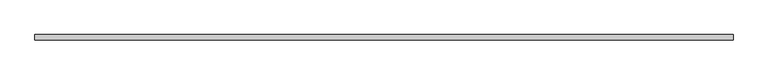
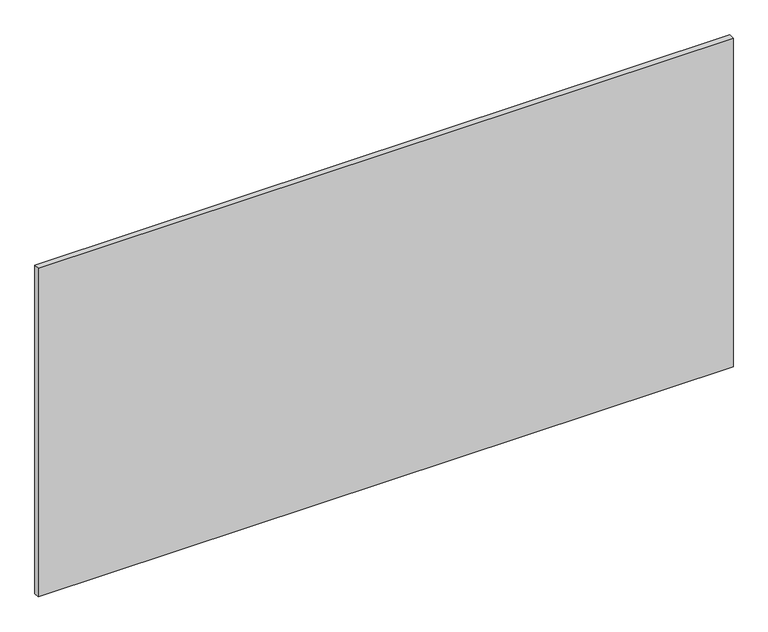
"""IFC4 building model written with IfcOpenShell, lengths in millimetres: proxy geometry, Inner panel:Inner panel:1:Inner panel:1 : Inner panel:Inner panel:300324:300043:Inner panel:1:Inner panel:1 : Inner panel:Inner panel:300324:300043 : Inner panel:Inner panel:1:Inner panel:1 : Inner panel:Inner panel:300324:300043:22 : Inner panel:Inner panel:1:Inner panel:1 : Inner panel:Inner panel:300324:300043:Inner panel:1:Inner panel:1 : Inner panel:Inner panel:300324:300043 : Inner panel:Inner panel:1:Inner panel:1 : Inner panel:Inner panel:300324:300043:300031."""

from ifc_helpers import new_model, si_unit, frame, origin, place, context, project, spatial, polyline, outline, extrude, source, transform, mapped, element, save


def generic_models_5df29abb(model_context):
    return source(origin(), model_context, "Body", "SweptSolid", [
        extrude(outline(polyline([(593738.0867239, -567913.5913841), (596176.4867239, -567913.5913841), (596176.4867239, -567932.6413841), (593738.0867239, -567932.6413841), (593738.0867239, -567913.5913841)])), frame((0.0, 0.0, 2495.55), z_axis=(0.0, 0.0, 1.0), x_axis=(1.0, 0.0, 0.0)), (0.0, 0.0, 1.0), 1219.2),
    ])


if __name__ == "__main__":
    model = new_model("IFC4")
    model_context = context("Model", 3, world=origin())
    ifc_project = project(units=[si_unit("LENGTHUNIT", "METRE", prefix="MILLI")], contexts=[model_context])
    site = spatial("IfcSite", under=ifc_project)
    building = spatial("IfcBuilding", under=site)
    placement = place(None, origin())
    generic_models_shape = generic_models_5df29abb(model_context)
    element("IfcBuildingElementProxy", 1, Name="Inner panel:Inner panel:1:Inner panel:1 : Inner panel:Inner panel:300324:300043:Inner panel:1:Inner panel:1 : Inner panel:Inner panel:300324:300043 : Inner panel:Inner panel:1:Inner panel:1 : Inner panel:Inner panel:300324:300043:22 : Inner panel:Inner panel:1:Inner panel:1 : Inner panel:Inner panel:300324:300043:Inner panel:1:Inner panel:1 : Inner panel:Inner panel:300324:300043 : Inner panel:Inner panel:1:Inner panel:1 : Inner panel:Inner panel:300324:300043:300031", ObjectType="Inner panel:Inner panel:1:Inner panel:1 : Inner panel:Inner panel:300324:300043:Inner panel:1:Inner panel:1 : Inner panel:Inner panel:300324:300043 : Inner panel:Inner panel:1:Inner panel:1 : Inner panel:Inner panel:300324:300043:22 : Inner panel:Inner panel:1:Inner panel:1 : Inner panel:Inner panel:300324:300043:Inner panel:1:Inner panel:1 : Inner panel:Inner panel:300324:300043 : Inner panel:Inner panel:1:Inner panel:1 : Inner panel:Inner panel:300324:300043:300031", at=placement, inside=building, context=model_context, shape_type="MappedRepresentation", body=[
        mapped(generic_models_shape, transform((0.0, 0.0, 0.0), x_axis=(1.0, 0.0, 0.0), y_axis=(0.0, 1.0, 0.0), z_axis=(0.0, 0.0, 1.0))),
    ])
    save(model, "model.ifc")

# Revit data of these elements
# Type "Inner panel:Inner panel:1:Inner panel:1 : Inner panel:Inner panel:300324:300043:Inner panel:1:Inner panel:1 : Inner panel:Inner panel:300324:300043 : Inner panel:Inner panel:1:Inner panel:1 : Inner panel:Inner panel:300324:300043:22 : Inner panel:Inner panel:1:Inner panel:1 : Inner panel:Inner panel:300324:300043:Inner panel:1:Inner panel:1 : Inner panel:Inner panel:300324:300043 : Inner panel:Inner panel:1:Inner panel:1 : Inner panel:Inner panel:300324:300043:300031"
#   NameOverride = "Inner panel:Inner panel:1:Inner panel:1 : Inner panel:Inner panel:300324:300043:Inner panel:1:Inner panel:1 : Inner panel:Inner panel:300324:300043 : Inner panel:Inner panel:1:Inner panel:1 : Inner panel:Inner panel:300324:300043:300031"
#   ObjectTypeOverride = "Inner panel:1:Inner panel:1 : Inner panel:Inner panel:300324:300043 : Inner panel:Inner panel:1:Inner panel:1 : Inner panel:Inner panel:300324:300043"
#   Reference = "Inner panel"
#   Tag = "300031"
# Element 1 (IfcBuildingElementProxy, "Inner panel:Inner panel:1:Inner panel:1 : Inner panel:Inner panel:300324:300043:Inner panel:1:Inner panel:1 : Inner panel:Inner panel:300324:300043 : Inner panel:Inner panel:1:Inner panel:1 : Inner panel:Inner panel:300324:300043:22 : Inner panel:Inner panel:1:Inner panel:1 : Inner panel:Inner panel:300324:300043:Inner panel:1:Inner panel:1 : Inner panel:Inner panel:300324:300043 : Inner panel:Inner panel:1:Inner panel:1 : Inner panel:Inner panel:300324:300043:300031")
#   Materials on its faces: "3/4\" PREFINISHED STAINED/SEALED PLYWOOD (FINISH: GRADE B,  FLAME SPREAD: CLASS B)"
# Materials
#   "3/4\" PREFINISHED STAINED/SEALED PLYWOOD (FINISH: GRADE B,  FLAME SPREAD: CLASS B)": class "Wood", colour RGB 149 120 74, transparency 0, Description = "Plywood, sheathing grade", Cost = 0
